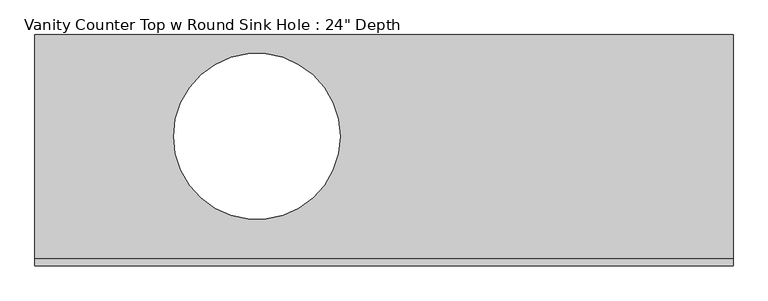
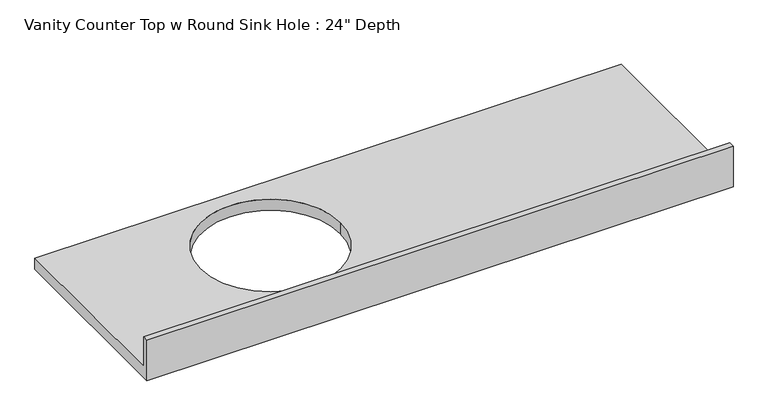
"""IFC4 building model written with IfcOpenShell, lengths in millimetres: furniture geometry."""

from ifc_helpers import new_model, si_unit, frame, origin, place, context, project, spatial, polyline, circle_curve, source, transform, mapped, element, save
from ifc_brep_helpers import plane_surface, revolved_surface, advanced_brep


def furniture_d9f50aac(model_context):
    return source(origin(), model_context, "Body", "AdvancedBrep", [
        advanced_brep(
        [(-1327.4622951, 635.0, 787.4), (-1327.4622951, 19.05, 787.4), (590.2377049, 19.05, 787.4), (590.2377049, 635.0, 787.4), (-489.2622951, 355.6, 787.4), (-946.4622951, 355.6, 787.4), (590.2377049, 0.0, 749.3), (-1327.4622951, 0.0, 749.3), (-1327.4622951, 635.0, 749.3), (590.2377049, 635.0, 749.3), (-946.4622951, 355.6, 749.3), (-489.2622951, 355.6, 749.3), (590.2377049, 0.0, 889.0), (-1327.4622951, 0.0, 889.0), (-1327.4622951, 19.05, 889.0), (590.2377049, 19.05, 889.0)],
        [
            (0, 1),
            (1, 2),
            (2, 3),
            (3, 0),
            (4, 5, circle_curve(frame((-717.8622951, 355.6, 787.4), z_axis=(0.0, 0.0, -1.0), x_axis=(1.0, 0.0, 0.0)), 228.6)),
            (5, 4, circle_curve(frame((-717.8622951, 355.6, 787.4), z_axis=(0.0, 0.0, -1.0), x_axis=(1.0, 0.0, 0.0)), 228.6)),
            (6, 7),
            (7, 8),
            (8, 9),
            (9, 6),
            (10, 11, circle_curve(frame((-717.8622951, 355.6, 749.3), z_axis=(0.0, 0.0, 1.0), x_axis=(1.0, 0.0, 0.0)), 228.6)),
            (11, 10, circle_curve(frame((-717.8622951, 355.6, 749.3), z_axis=(0.0, 0.0, 1.0), x_axis=(1.0, 0.0, 0.0)), 228.6)),
            (6, 12),
            (12, 13),
            (13, 7),
            (13, 14),
            (14, 1),
            (0, 8),
            (3, 9),
            (2, 15),
            (15, 12),
            (15, 14),
            (5, 10),
            (11, 4),
        ],
        [
            plane_surface(frame((-1327.4622951, 0.0, 787.4), z_axis=(0.0, 0.0, 1.0), x_axis=(-1.0, 0.0, 0.0))),
            plane_surface(frame((-1327.4622951, 0.0, 749.3), z_axis=(0.0, 0.0, -1.0), x_axis=(1.0, 0.0, 0.0))),
            plane_surface(frame((590.2377049, 0.0, 787.4), z_axis=(0.0, -1.0, 0.0), x_axis=(0.0, 0.0, -1.0))),
            plane_surface(frame((-1327.4622951, 0.0, 787.4), z_axis=(-1.0, 0.0, 0.0), x_axis=(0.0, 0.0, -1.0))),
            plane_surface(frame((-1327.4622951, 635.0, 787.4), z_axis=(0.0, 1.0, 0.0), x_axis=(0.0, 0.0, -1.0))),
            plane_surface(frame((590.2377049, 635.0, 787.4), z_axis=(1.0, 0.0, 0.0), x_axis=(0.0, 0.0, -1.0))),
            plane_surface(frame((-1327.4622951, 0.0, 889.0), z_axis=(0.0, 0.0, 1.0), x_axis=(0.0, 1.0, 0.0))),
            plane_surface(frame((-1327.4622951, 19.05, 889.0), z_axis=(0.0, 1.0, 0.0), x_axis=(0.0, 0.0, -1.0))),
            revolved_surface(polyline([(-489.26229509999996, 355.6, 787.4), (-489.26229509999996, 355.6, 749.3)]), (-717.8622951, 355.6, 749.3), (0.0, 0.0, 1.0)),
        ],
        [
            (0, [[1, 2, 3, 4], [5, 6]]),
            (1, [[7, 8, 9, 10], [11, 12]]),
            (2, [[13, 14, 15, -7]]),
            (3, [[-15, 16, 17, -1, 18, -8]]),
            (4, [[19, -9, -18, -4]]),
            (5, [[-19, -3, 20, 21, -13, -10]]),
            (6, [[-14, -21, 22, -16]]),
            (7, [[-20, -2, -17, -22]]),
            (8, [[-6, 23, -12, 24]]),
            (8, [[-11, -23, -5, -24]]),
        ],
    ),
    ])


if __name__ == "__main__":
    model = new_model("IFC4")
    model_context = context("Model", 3, world=origin())
    ifc_project = project(units=[si_unit("LENGTHUNIT", "METRE", prefix="MILLI")], contexts=[model_context])
    site = spatial("IfcSite", under=ifc_project)
    building = spatial("IfcBuilding", under=site)
    placement = place(None, origin())
    furniture_shape = furniture_d9f50aac(model_context)
    element("IfcFurniture", 1, ObjectType="Vanity Counter Top w Round Sink Hole : 24\" Depth", at=placement, inside=building, context=model_context, shape_type="MappedRepresentation", body=[
        mapped(furniture_shape, transform((0.0, 0.0, 0.0), x_axis=(1.0, 0.0, 0.0), y_axis=(0.0, 1.0, 0.0), z_axis=(0.0, 0.0, 1.0))),
    ])
    save(model, "model.ifc")

# Revit data of these elements
# Type "Vanity Counter Top w Round Sink Hole : 24\" Depth"
#   Assembly Code = "C1030400"
#   Counter Thickness = 0' - 1 1/2"
#   Depth = 2' - 1"
#   Height = 2' - 7"
#   Length [instance default] = 4' - 0"
#   Sink Location [instance default] = 2' - 0"
#   Sink Location To Wall [instance default] = 0' - 4"
#   Sink Opening Width [instance default] = 1' - 5"
#   Counter Top Material = Laminate, Blue, Matte
#   Default Elevation = 0
# Element 1 (IfcFurniture, "Vanity Counter Top w Round Sink Hole : 24\" Depth")
#   Length = 6' - 3 1/2"
#   Sink Location To Wall = 0' - 5 1/2"
#   Materials on its faces: "Laminate, Blue, Matte"
# Materials
#   "Laminate, Blue, Matte": class "Plastic", colour RGB 85 101 155, transparency 0, Description = "Plastic Laminate - Blue, Matte", Cost = 0
